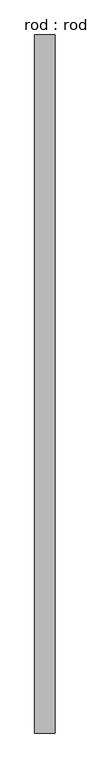
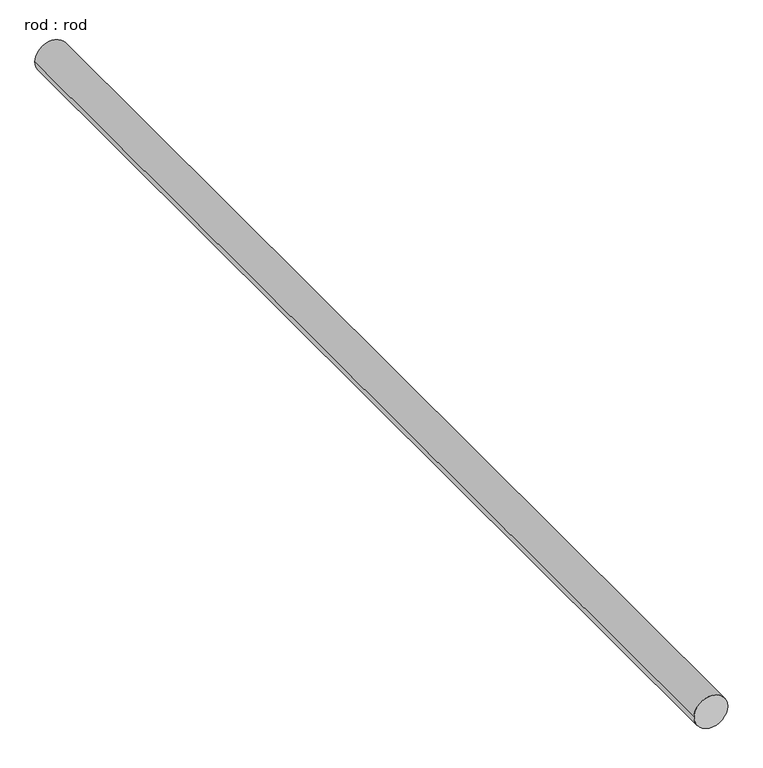
"""IFC4 building model written with IfcOpenShell, lengths in millimetres: proxy geometry, rod : rod."""

from ifc_helpers import new_model, si_unit, point, frame, frame_2d, origin, place, context, project, spatial, circle_curve, trimmed, segment, composite_curve, outline, extrude, source, transform, mapped, element, save


def rod_rod_8db86969(model_context):
    return source(origin(), model_context, "Body", "SweptSolid", [
        extrude(outline(composite_curve([segment(trimmed(circle_curve(frame_2d((0.0108462, 0.0)), 200.0), [point((0.0108462, 200.0))], [point((0.0108462, -200.0))], False, "CARTESIAN"), True, "CONTINUOUS"), segment(trimmed(circle_curve(frame_2d((0.0108462, 0.0)), 200.0), [point((0.0108462, -200.0))], [point((0.0108462, 200.0))], False, "CARTESIAN"), True, "CONTINUOUS")], self_intersect=False)), frame((0.0, -2714.5634459, 0.0), z_axis=(0.0, 1.0, 0.0), x_axis=(0.0, 0.0, 1.0)), (0.0, 0.0, 1.0), 13614.5841224),
    ])


if __name__ == "__main__":
    model = new_model("IFC4")
    model_context = context("Model", 3, world=origin())
    ifc_project = project(units=[si_unit("LENGTHUNIT", "METRE", prefix="MILLI")], contexts=[model_context])
    site = spatial("IfcSite", under=ifc_project)
    building = spatial("IfcBuilding", under=site)
    placement = place(None, origin())
    rod_rod_shape = rod_rod_8db86969(model_context)
    element("IfcBuildingElementProxy", 1, Name="rod : rod", ObjectType="rod : rod", at=placement, inside=building, context=model_context, shape_type="MappedRepresentation", body=[
        mapped(rod_rod_shape, transform((0.0, 0.0, 0.0), x_axis=(1.0, 0.0, 0.0), y_axis=(0.0, 1.0, 0.0), z_axis=(0.0, 0.0, 1.0))),
    ])
    save(model, "model.ifc")

# Revit data of these elements
# Type "rod : rod"
#   Default Elevation = 0
